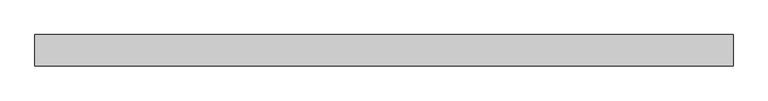
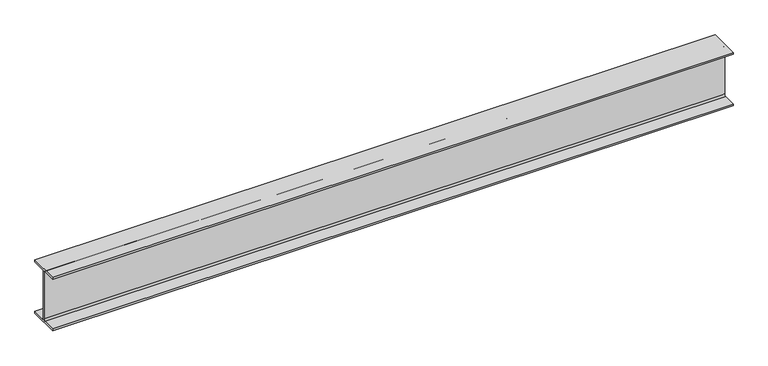
"""IFC4 building model written with IfcOpenShell, lengths in millimetres: beam geometry, Old_Steel Beam_H-KSD3502 : H_SB_ASB_H-200×200x8x12."""

import ifcopenshell
import ifcopenshell.guid

model = None  # the IFC model being written
_history = None  # IfcOwnerHistory: only IFC2X3 demands one
_inside = {}  # id of a spatial element -> (the spatial element, [elements in it])
_under = {}  # id of a project, library or spatial element -> (it, [spatial elements below it])
_declared = {}  # id of a project -> (the project, [libraries it declares])
_typed = {}  # id of a type object -> (the type object, [elements of that type])
_made_of = {}  # id of a material, layer set ... -> (it, [elements and type objects made of it])


def new_model(schema):
    """Start an empty IFC model of exactly this schema.

    Asked for "IFC4X3", IfcOpenShell would pick the latest addendum, in which some entities
    have other attributes; the version numbers below select the first issue.
    IFC2X3 requires an IfcOwnerHistory on every rooted entity: one is made here for all.
    """
    global model, _history
    if schema == "IFC4X3":
        model = ifcopenshell.file(schema_version=(4, 3, 0, 0))
    else:
        model = ifcopenshell.file(schema=schema)
    _inside.clear()
    _under.clear()
    _declared.clear()
    _typed.clear()
    _made_of.clear()
    _history = None
    if model.schema == "IFC2X3":
        org = make("IfcOrganization", Name="unknown")
        user = make(
            "IfcPersonAndOrganization",
            ThePerson=make("IfcPerson", FamilyName="unknown"),
            TheOrganization=org,
        )
        app = make(
            "IfcApplication",
            ApplicationDeveloper=org,
            Version="unknown",
            ApplicationFullName="unknown",
            ApplicationIdentifier="unknown",
        )
        _history = make(
            "IfcOwnerHistory",
            OwningUser=user,
            OwningApplication=app,
            ChangeAction="ADDED",
            CreationDate=0,
        )
    return model


def make(cls, **values):
    """One entity of the class cls with the attributes given. An attribute that is None is left unset."""
    return model.create_entity(
        cls, **{name: value for name, value in values.items() if value is not None}
    )


def rooted(cls, **values):
    """An entity with a GlobalId (a new one), such as an element, a storey or a relation."""
    return make(cls, GlobalId=ifcopenshell.guid.new(), OwnerHistory=_history, **values)


def si_unit(unit_type, name, prefix=None):
    """IfcSIUnit, for example si_unit("LENGTHUNIT", "METRE", prefix="MILLI")."""
    return make("IfcSIUnit", UnitType=unit_type, Prefix=prefix, Name=name)


def assignment(units):
    """IfcUnitAssignment: the units of a project."""
    return None if units is None else make("IfcUnitAssignment", Units=units)


def point(xyz):
    """IfcCartesianPoint."""
    return None if xyz is None else make("IfcCartesianPoint", Coordinates=xyz)


def direction(xyz):
    """IfcDirection."""
    return None if xyz is None else make("IfcDirection", DirectionRatios=xyz)


def frame(location, z_axis=None, x_axis=None):
    """IfcAxis2Placement3D, a coordinate frame: its origin and axes. An axis left out is left unset."""
    return make(
        "IfcAxis2Placement3D",
        Location=point(location),
        Axis=direction(z_axis),
        RefDirection=direction(x_axis),
    )


def frame_2d(location, x_axis=None):
    """IfcAxis2Placement2D, a coordinate frame in the plane: its origin and x axis."""
    return make(
        "IfcAxis2Placement2D", Location=point(location), RefDirection=direction(x_axis)
    )


def origin():
    """The frame at (0, 0, 0) with its axes left unset."""
    return frame((0.0, 0.0, 0.0))


def place(relative_to, where):
    """IfcLocalPlacement: puts the frame where relative to a parent placement (None: the world)."""
    return make(
        "IfcLocalPlacement", PlacementRelTo=relative_to, RelativePlacement=where
    )


def context(
    kind, dimensions, precision=None, world=None, true_north=None, identifier=None
):
    """IfcGeometricRepresentationContext, for example the 3D "Model" context."""
    return make(
        "IfcGeometricRepresentationContext",
        ContextIdentifier=identifier,
        ContextType=kind,
        CoordinateSpaceDimension=dimensions,
        Precision=precision,
        WorldCoordinateSystem=world,
        TrueNorth=true_north,
    )


def project(units=None, contexts=None):
    """IfcProject with its units and contexts."""
    return rooted(
        "IfcProject",
        Name="project",
        RepresentationContexts=contexts,
        UnitsInContext=assignment(units),
    )


def spatial(cls, under=None, at=None, **own):
    """A site, building, storey or space (cls), placed at a placement, below another one or the project."""
    s = rooted(cls, ObjectPlacement=at, **own)
    if under is not None:
        _under.setdefault(under.id(), (under, []))[1].append(s)
    return s


def polyline(points):
    """IfcPolyline through the points."""
    return make("IfcPolyline", Points=[point(p) for p in points])


def circle_curve(where, radius):
    """IfcCircle in the frame where."""
    return make("IfcCircle", Position=where, Radius=radius)


def trimmed(basis, trim1, trim2, sense, master):
    """IfcTrimmedCurve: the piece of a basis curve between two trims."""
    return make(
        "IfcTrimmedCurve",
        BasisCurve=basis,
        Trim1=trim1,
        Trim2=trim2,
        SenseAgreement=sense,
        MasterRepresentation=master,
    )


def segment(curve, same_sense, transition):
    """IfcCompositeCurveSegment."""
    return make(
        "IfcCompositeCurveSegment",
        Transition=transition,
        SameSense=same_sense,
        ParentCurve=curve,
    )


def composite_curve(segments, self_intersect=None):
    """IfcCompositeCurve: segments joined end to end."""
    return make("IfcCompositeCurve", Segments=segments, SelfIntersect=self_intersect)


def outline(outer, holes=None, kind="AREA"):
    """IfcArbitraryClosedProfileDef: a profile drawn as a closed curve; with holes, ...WithVoids."""
    if holes is None:
        return make("IfcArbitraryClosedProfileDef", ProfileType=kind, OuterCurve=outer)
    return make(
        "IfcArbitraryProfileDefWithVoids",
        ProfileType=kind,
        OuterCurve=outer,
        InnerCurves=holes,
    )


def extrude(swept, where, along, depth):
    """IfcExtrudedAreaSolid: the profile swept, set in the frame where, extruded along a direction by depth."""
    return make(
        "IfcExtrudedAreaSolid",
        SweptArea=swept,
        Position=where,
        ExtrudedDirection=direction(along),
        Depth=depth,
    )


def shape(context_of_items, identifier, shape_type, items):
    """IfcShapeRepresentation: the items that make up one representation, for example the "Body"."""
    return make(
        "IfcShapeRepresentation",
        ContextOfItems=context_of_items,
        RepresentationIdentifier=identifier,
        RepresentationType=shape_type,
        Items=items,
    )


def source(mapping_origin, context_of_items, identifier, shape_type, items):
    """IfcRepresentationMap: a shape defined once, which mapped items show again and again."""
    return make(
        "IfcRepresentationMap",
        MappingOrigin=mapping_origin,
        MappedRepresentation=shape(context_of_items, identifier, shape_type, items),
    )


def transform(
    local_origin,
    x_axis=None,
    y_axis=None,
    z_axis=None,
    scale=None,
    scale2=None,
    scale3=None,
    uniform=True,
):
    """IfcCartesianTransformationOperator3D, or its non-uniform kind. x_axis, y_axis, z_axis: its Axis1, 2, 3."""
    if uniform:
        return make(
            "IfcCartesianTransformationOperator3D",
            Axis1=direction(x_axis),
            Axis2=direction(y_axis),
            LocalOrigin=point(local_origin),
            Scale=scale,
            Axis3=direction(z_axis),
        )
    return make(
        "IfcCartesianTransformationOperator3DnonUniform",
        Axis1=direction(x_axis),
        Axis2=direction(y_axis),
        LocalOrigin=point(local_origin),
        Scale=scale,
        Axis3=direction(z_axis),
        Scale2=scale2,
        Scale3=scale3,
    )


def mapped(mapping_source, mapping_target):
    """IfcMappedItem: shows the shape of a source again, moved by a transform."""
    return make(
        "IfcMappedItem", MappingSource=mapping_source, MappingTarget=mapping_target
    )


def made_of(thing, what):
    """Note that an element or type object is made of a material, layer set ...; save() writes the relation."""
    if what is not None:
        _made_of.setdefault(what.id(), (what, []))[1].append(thing)
    return thing


def element(
    cls,
    number,
    at=None,
    inside=None,
    cuts=None,
    type_object=None,
    material=None,
    context=None,
    identifier="Body",
    shape_type=None,
    held_by="IfcProductDefinitionShape",
    body=None,
    shapes=None,
    **own,
):
    """One element of the class cls, such as IfcWall. Its Tag is "e" and its number.

    at: its placement. inside: the storey or other place that contains it. cuts: it is an
    opening in that element (IfcRelVoidsElement). A single representation is given by context,
    identifier, shape_type and body (its items); several are given by shapes. held_by: the class
    of the entity that holds the representations. save() writes the other relations.
    """
    e = rooted(cls, Tag="e%d" % number, ObjectPlacement=at, **own)
    if body is not None:
        shapes = [shape(context, identifier, shape_type, body)]
    if shapes is not None:
        e.Representation = make(held_by, Representations=shapes)
    if inside is not None:
        _inside.setdefault(inside.id(), (inside, []))[1].append(e)
    if cuts is not None:
        rooted(
            "IfcRelVoidsElement", RelatingBuildingElement=cuts, RelatedOpeningElement=e
        )
    if type_object is not None:
        _typed.setdefault(type_object.id(), (type_object, []))[1].append(e)
    return made_of(e, material)


def aggregate(whole, parts):
    """IfcRelAggregates: a whole, such as a stair, and the parts it consists of."""
    return rooted("IfcRelAggregates", RelatingObject=whole, RelatedObjects=parts)


def save(model, path):
    """Write the relations noted so far, then the file.

    IfcRelAggregates (storeys below a building ...), IfcRelContainedInSpatialStructure (elements
    in a storey), IfcRelDefinesByType, IfcRelAssociatesMaterial and IfcRelDeclares: one each for
    every whole, place, type object, material and project.
    """
    for whole, parts in _under.values():
        aggregate(whole, parts)
    for where, things in _inside.values():
        rooted(
            "IfcRelContainedInSpatialStructure",
            RelatedElements=things,
            RelatingStructure=where,
        )
    for kind, things in _typed.values():
        rooted("IfcRelDefinesByType", RelatedObjects=things, RelatingType=kind)
    for what, things in _made_of.values():
        rooted("IfcRelAssociatesMaterial", RelatedObjects=things, RelatingMaterial=what)
    for by, libraries in _declared.values():
        rooted("IfcRelDeclares", RelatingContext=by, RelatedDefinitions=libraries)
    model.write(path)


def beam_298d0fa7(model_context):
    return source(origin(), model_context, "Body", "SweptSolid", [
        extrude(outline(composite_curve([segment(polyline([(-82.5, -141.5), (-11.9, -141.5)]), True, "CONTINUOUS"), segment(trimmed(circle_curve(frame_2d((-11.9, -132.6)), 8.9), [point((-11.9, -141.5))], [point((-3.0, -132.6))], True, "CARTESIAN"), True, "CONTINUOUS"), segment(polyline([(-3.0, -132.6), (-3.0, 132.6)]), True, "CONTINUOUS"), segment(trimmed(circle_curve(frame_2d((-11.9, 132.6)), 8.9), [point((-3.0, 132.6))], [point((-11.9, 141.5))], True, "CARTESIAN"), True, "CONTINUOUS"), segment(polyline([(-11.9, 141.5), (-82.5, 141.5), (-82.5, 151.7), (82.5, 151.7), (82.5, 141.5), (11.9, 141.5)]), True, "CONTINUOUS"), segment(trimmed(circle_curve(frame_2d((11.9, 132.6)), 8.9), [point((11.9, 141.5))], [point((3.0, 132.6))], True, "CARTESIAN"), True, "CONTINUOUS"), segment(polyline([(3.0, 132.6), (3.0, -132.6)]), True, "CONTINUOUS"), segment(trimmed(circle_curve(frame_2d((11.9, -132.6)), 8.9), [point((3.0, -132.6))], [point((11.9, -141.5))], True, "CARTESIAN"), True, "CONTINUOUS"), segment(polyline([(11.9, -141.5), (82.5, -141.5), (82.5, -151.7), (-82.5, -151.7), (-82.5, -141.5)]), True, "CONTINUOUS")], self_intersect=False)), frame((-1840.6096779, 0.0, 0.0), z_axis=(1.0, 0.0, 0.0), x_axis=(0.0, 1.0, 0.0)), (0.0, 0.0, 1.0), 3657.360877),
    ])


if __name__ == "__main__":
    model = new_model("IFC4")
    model_context = context("Model", 3, world=origin())
    ifc_project = project(units=[si_unit("LENGTHUNIT", "METRE", prefix="MILLI")], contexts=[model_context])
    site = spatial("IfcSite", under=ifc_project)
    building = spatial("IfcBuilding", under=site)
    placement = place(None, origin())
    beam_shape = beam_298d0fa7(model_context)
    element("IfcBeam", 1, ObjectType="Old_Steel Beam_H-KSD3502 : H_SB_ASB_H-200×200x8x12", at=placement, inside=building, context=model_context, shape_type="MappedRepresentation", body=[
        mapped(beam_shape, transform((0.0, 0.0, 0.0), x_axis=(1.0, 0.0, 0.0), y_axis=(0.0, 1.0, 0.0), z_axis=(0.0, 0.0, 1.0))),
    ])
    save(model, "model.ifc")

# Revit data of these elements
# Type "Old_Steel Beam_H-KSD3502 : H_SB_ASB_H-200×200x8x12"
#   Width = 20.0 cm
#   Web Thickness = 0.8 cm
#   Web Fillet = 1.3 cm
#   Warping Constant = 141376.0 cm⁶
#   Torsional Moment of Inertia = 26.2485 cm⁴
#   Torsional Modulus = 1.0 cm³
#   Section Area = 63.53 cm²
#   Plastic Modulus weak axis = 244.0 cm³
#   Plastic Modulus strong axis = 525.0 cm³
#   Perimeter = 1.16 m²/m
#   Nominal Weight = 49.90 kgf/m
#   Moment of Inertia weak axis = 1600.00 cm⁴
#   Moment of Inertia strong axis = 4720.00 cm⁴
#   Height = 20.0 cm
#   Flange Thickness = 1.2 cm
#   Elastic Modulus weak axis = 160.0 cm³
#   Elastic Modulus strong axis = 472.0 cm³
#   Centroid Vertical = 10.0 cm
#   Centroid Horizontal = 10.0 cm
#   Length [instance default] = 1.5240 m
#   Structural Material [instance default] = Steel, 45-345
#   Assembly Code = ""
# Element 1 (IfcBeam, "Old_Steel Beam_H-KSD3502 : H_SB_ASB_H-200×200x8x12")
#   Structural Material = none
# Materials
#   "Steel, 45-345": class "Metal", colour RGB 189 187 185, transparency 0, Description = "Steel 345 MPa", Cost = 0
